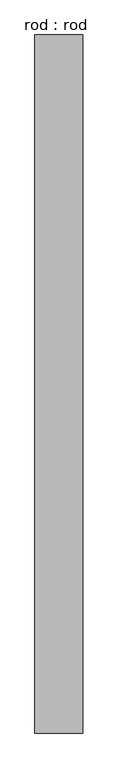
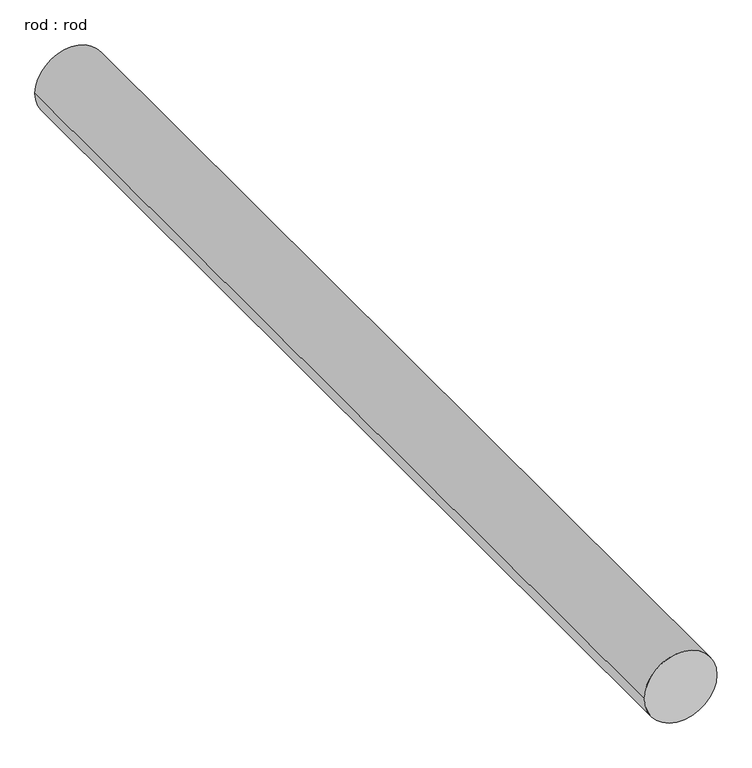
"""IFC4 building model written with IfcOpenShell, lengths in millimetres: proxy geometry, rod : rod."""

import ifcopenshell
import ifcopenshell.guid

model = None  # the IFC model being written
_history = None  # IfcOwnerHistory: only IFC2X3 demands one
_inside = {}  # id of a spatial element -> (the spatial element, [elements in it])
_under = {}  # id of a project, library or spatial element -> (it, [spatial elements below it])
_declared = {}  # id of a project -> (the project, [libraries it declares])
_typed = {}  # id of a type object -> (the type object, [elements of that type])
_made_of = {}  # id of a material, layer set ... -> (it, [elements and type objects made of it])


def new_model(schema):
    """Start an empty IFC model of exactly this schema.

    Asked for "IFC4X3", IfcOpenShell would pick the latest addendum, in which some entities
    have other attributes; the version numbers below select the first issue.
    IFC2X3 requires an IfcOwnerHistory on every rooted entity: one is made here for all.
    """
    global model, _history
    if schema == "IFC4X3":
        model = ifcopenshell.file(schema_version=(4, 3, 0, 0))
    else:
        model = ifcopenshell.file(schema=schema)
    _inside.clear()
    _under.clear()
    _declared.clear()
    _typed.clear()
    _made_of.clear()
    _history = None
    if model.schema == "IFC2X3":
        org = make("IfcOrganization", Name="unknown")
        user = make(
            "IfcPersonAndOrganization",
            ThePerson=make("IfcPerson", FamilyName="unknown"),
            TheOrganization=org,
        )
        app = make(
            "IfcApplication",
            ApplicationDeveloper=org,
            Version="unknown",
            ApplicationFullName="unknown",
            ApplicationIdentifier="unknown",
        )
        _history = make(
            "IfcOwnerHistory",
            OwningUser=user,
            OwningApplication=app,
            ChangeAction="ADDED",
            CreationDate=0,
        )
    return model


def make(cls, **values):
    """One entity of the class cls with the attributes given. An attribute that is None is left unset."""
    return model.create_entity(
        cls, **{name: value for name, value in values.items() if value is not None}
    )


def rooted(cls, **values):
    """An entity with a GlobalId (a new one), such as an element, a storey or a relation."""
    return make(cls, GlobalId=ifcopenshell.guid.new(), OwnerHistory=_history, **values)


def si_unit(unit_type, name, prefix=None):
    """IfcSIUnit, for example si_unit("LENGTHUNIT", "METRE", prefix="MILLI")."""
    return make("IfcSIUnit", UnitType=unit_type, Prefix=prefix, Name=name)


def assignment(units):
    """IfcUnitAssignment: the units of a project."""
    return None if units is None else make("IfcUnitAssignment", Units=units)


def point(xyz):
    """IfcCartesianPoint."""
    return None if xyz is None else make("IfcCartesianPoint", Coordinates=xyz)


def direction(xyz):
    """IfcDirection."""
    return None if xyz is None else make("IfcDirection", DirectionRatios=xyz)


def frame(location, z_axis=None, x_axis=None):
    """IfcAxis2Placement3D, a coordinate frame: its origin and axes. An axis left out is left unset."""
    return make(
        "IfcAxis2Placement3D",
        Location=point(location),
        Axis=direction(z_axis),
        RefDirection=direction(x_axis),
    )


def frame_2d(location, x_axis=None):
    """IfcAxis2Placement2D, a coordinate frame in the plane: its origin and x axis."""
    return make(
        "IfcAxis2Placement2D", Location=point(location), RefDirection=direction(x_axis)
    )


def origin():
    """The frame at (0, 0, 0) with its axes left unset."""
    return frame((0.0, 0.0, 0.0))


def place(relative_to, where):
    """IfcLocalPlacement: puts the frame where relative to a parent placement (None: the world)."""
    return make(
        "IfcLocalPlacement", PlacementRelTo=relative_to, RelativePlacement=where
    )


def context(
    kind, dimensions, precision=None, world=None, true_north=None, identifier=None
):
    """IfcGeometricRepresentationContext, for example the 3D "Model" context."""
    return make(
        "IfcGeometricRepresentationContext",
        ContextIdentifier=identifier,
        ContextType=kind,
        CoordinateSpaceDimension=dimensions,
        Precision=precision,
        WorldCoordinateSystem=world,
        TrueNorth=true_north,
    )


def project(units=None, contexts=None):
    """IfcProject with its units and contexts."""
    return rooted(
        "IfcProject",
        Name="project",
        RepresentationContexts=contexts,
        UnitsInContext=assignment(units),
    )


def spatial(cls, under=None, at=None, **own):
    """A site, building, storey or space (cls), placed at a placement, below another one or the project."""
    s = rooted(cls, ObjectPlacement=at, **own)
    if under is not None:
        _under.setdefault(under.id(), (under, []))[1].append(s)
    return s


def circle_curve(where, radius):
    """IfcCircle in the frame where."""
    return make("IfcCircle", Position=where, Radius=radius)


def trimmed(basis, trim1, trim2, sense, master):
    """IfcTrimmedCurve: the piece of a basis curve between two trims."""
    return make(
        "IfcTrimmedCurve",
        BasisCurve=basis,
        Trim1=trim1,
        Trim2=trim2,
        SenseAgreement=sense,
        MasterRepresentation=master,
    )


def segment(curve, same_sense, transition):
    """IfcCompositeCurveSegment."""
    return make(
        "IfcCompositeCurveSegment",
        Transition=transition,
        SameSense=same_sense,
        ParentCurve=curve,
    )


def composite_curve(segments, self_intersect=None):
    """IfcCompositeCurve: segments joined end to end."""
    return make("IfcCompositeCurve", Segments=segments, SelfIntersect=self_intersect)


def outline(outer, holes=None, kind="AREA"):
    """IfcArbitraryClosedProfileDef: a profile drawn as a closed curve; with holes, ...WithVoids."""
    if holes is None:
        return make("IfcArbitraryClosedProfileDef", ProfileType=kind, OuterCurve=outer)
    return make(
        "IfcArbitraryProfileDefWithVoids",
        ProfileType=kind,
        OuterCurve=outer,
        InnerCurves=holes,
    )


def extrude(swept, where, along, depth):
    """IfcExtrudedAreaSolid: the profile swept, set in the frame where, extruded along a direction by depth."""
    return make(
        "IfcExtrudedAreaSolid",
        SweptArea=swept,
        Position=where,
        ExtrudedDirection=direction(along),
        Depth=depth,
    )


def shape(context_of_items, identifier, shape_type, items):
    """IfcShapeRepresentation: the items that make up one representation, for example the "Body"."""
    return make(
        "IfcShapeRepresentation",
        ContextOfItems=context_of_items,
        RepresentationIdentifier=identifier,
        RepresentationType=shape_type,
        Items=items,
    )


def source(mapping_origin, context_of_items, identifier, shape_type, items):
    """IfcRepresentationMap: a shape defined once, which mapped items show again and again."""
    return make(
        "IfcRepresentationMap",
        MappingOrigin=mapping_origin,
        MappedRepresentation=shape(context_of_items, identifier, shape_type, items),
    )


def transform(
    local_origin,
    x_axis=None,
    y_axis=None,
    z_axis=None,
    scale=None,
    scale2=None,
    scale3=None,
    uniform=True,
):
    """IfcCartesianTransformationOperator3D, or its non-uniform kind. x_axis, y_axis, z_axis: its Axis1, 2, 3."""
    if uniform:
        return make(
            "IfcCartesianTransformationOperator3D",
            Axis1=direction(x_axis),
            Axis2=direction(y_axis),
            LocalOrigin=point(local_origin),
            Scale=scale,
            Axis3=direction(z_axis),
        )
    return make(
        "IfcCartesianTransformationOperator3DnonUniform",
        Axis1=direction(x_axis),
        Axis2=direction(y_axis),
        LocalOrigin=point(local_origin),
        Scale=scale,
        Axis3=direction(z_axis),
        Scale2=scale2,
        Scale3=scale3,
    )


def mapped(mapping_source, mapping_target):
    """IfcMappedItem: shows the shape of a source again, moved by a transform."""
    return make(
        "IfcMappedItem", MappingSource=mapping_source, MappingTarget=mapping_target
    )


def made_of(thing, what):
    """Note that an element or type object is made of a material, layer set ...; save() writes the relation."""
    if what is not None:
        _made_of.setdefault(what.id(), (what, []))[1].append(thing)
    return thing


def element(
    cls,
    number,
    at=None,
    inside=None,
    cuts=None,
    type_object=None,
    material=None,
    context=None,
    identifier="Body",
    shape_type=None,
    held_by="IfcProductDefinitionShape",
    body=None,
    shapes=None,
    **own,
):
    """One element of the class cls, such as IfcWall. Its Tag is "e" and its number.

    at: its placement. inside: the storey or other place that contains it. cuts: it is an
    opening in that element (IfcRelVoidsElement). A single representation is given by context,
    identifier, shape_type and body (its items); several are given by shapes. held_by: the class
    of the entity that holds the representations. save() writes the other relations.
    """
    e = rooted(cls, Tag="e%d" % number, ObjectPlacement=at, **own)
    if body is not None:
        shapes = [shape(context, identifier, shape_type, body)]
    if shapes is not None:
        e.Representation = make(held_by, Representations=shapes)
    if inside is not None:
        _inside.setdefault(inside.id(), (inside, []))[1].append(e)
    if cuts is not None:
        rooted(
            "IfcRelVoidsElement", RelatingBuildingElement=cuts, RelatedOpeningElement=e
        )
    if type_object is not None:
        _typed.setdefault(type_object.id(), (type_object, []))[1].append(e)
    return made_of(e, material)


def aggregate(whole, parts):
    """IfcRelAggregates: a whole, such as a stair, and the parts it consists of."""
    return rooted("IfcRelAggregates", RelatingObject=whole, RelatedObjects=parts)


def save(model, path):
    """Write the relations noted so far, then the file.

    IfcRelAggregates (storeys below a building ...), IfcRelContainedInSpatialStructure (elements
    in a storey), IfcRelDefinesByType, IfcRelAssociatesMaterial and IfcRelDeclares: one each for
    every whole, place, type object, material and project.
    """
    for whole, parts in _under.values():
        aggregate(whole, parts)
    for where, things in _inside.values():
        rooted(
            "IfcRelContainedInSpatialStructure",
            RelatedElements=things,
            RelatingStructure=where,
        )
    for kind, things in _typed.values():
        rooted("IfcRelDefinesByType", RelatedObjects=things, RelatingType=kind)
    for what, things in _made_of.values():
        rooted("IfcRelAssociatesMaterial", RelatedObjects=things, RelatingMaterial=what)
    for by, libraries in _declared.values():
        rooted("IfcRelDeclares", RelatingContext=by, RelatedDefinitions=libraries)
    model.write(path)


def rod_rod_debf6b8e(model_context):
    return source(origin(), model_context, "Body", "SweptSolid", [
        extrude(outline(composite_curve([segment(trimmed(circle_curve(frame_2d((0.0108462, 0.0)), 200.0), [point((0.0108462, 200.0))], [point((0.0108462, -200.0))], False, "CARTESIAN"), True, "CONTINUOUS"), segment(trimmed(circle_curve(frame_2d((0.0108462, 0.0)), 200.0), [point((0.0108462, -200.0))], [point((0.0108462, 200.0))], False, "CARTESIAN"), True, "CONTINUOUS")], self_intersect=False)), frame((0.0, 1188.7070849, 0.0), z_axis=(0.0, 1.0, 0.0), x_axis=(0.0, 0.0, 1.0)), (0.0, 0.0, 1.0), 5808.0430609),
    ])


if __name__ == "__main__":
    model = new_model("IFC4")
    model_context = context("Model", 3, world=origin())
    ifc_project = project(units=[si_unit("LENGTHUNIT", "METRE", prefix="MILLI")], contexts=[model_context])
    site = spatial("IfcSite", under=ifc_project)
    building = spatial("IfcBuilding", under=site)
    placement = place(None, origin())
    rod_rod_shape = rod_rod_debf6b8e(model_context)
    element("IfcBuildingElementProxy", 1, Name="rod : rod", ObjectType="rod : rod", at=placement, inside=building, context=model_context, shape_type="MappedRepresentation", body=[
        mapped(rod_rod_shape, transform((0.0, 0.0, 0.0), x_axis=(1.0, 0.0, 0.0), y_axis=(0.0, 1.0, 0.0), z_axis=(0.0, 0.0, 1.0))),
    ])
    save(model, "model.ifc")

# Revit data of these elements
# Type "rod : rod"
#   Default Elevation = 0
